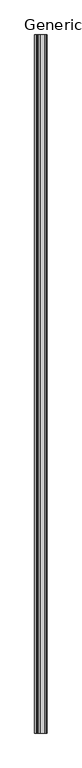
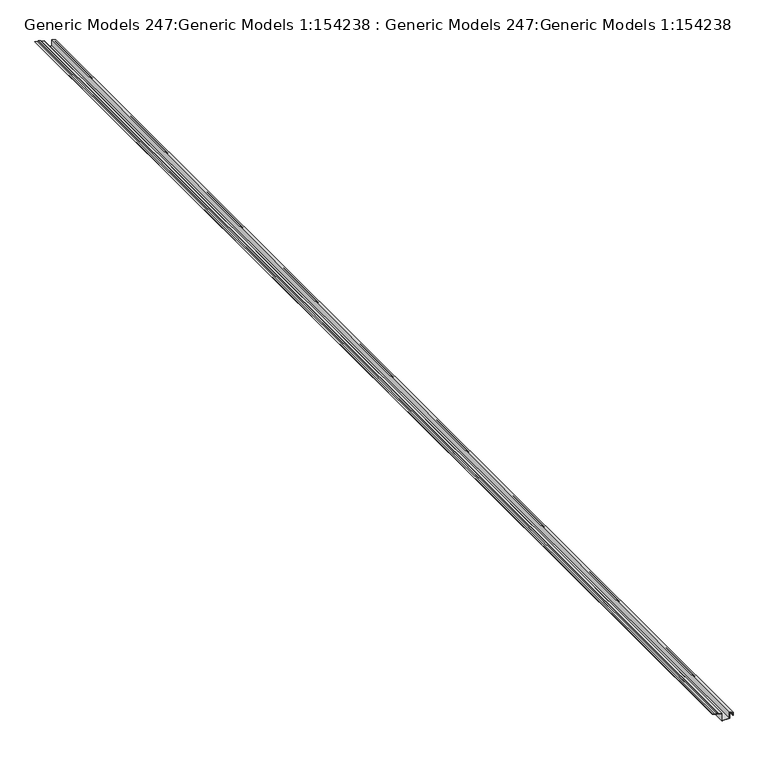
"""IFC4 building model written with IfcOpenShell, lengths in millimetres: proxy geometry, Generic Models 247:Generic Models 1:154238 : Generic Models 247:Generic Models 1:154238."""

from ifc_helpers import new_model, si_unit, point, frame, frame_2d, origin, place, context, project, spatial, polyline, circle_curve, trimmed, segment, composite_curve, outline, extrude, source, transform, mapped, element, save


def generic_models_247_generic_models_1_154238_generic_models_f81f4326(model_context):
    return source(origin(), model_context, "Body", "SweptSolid", [
        extrude(outline(polyline([(6352.8619087, 2093.6944594), (6358.1032399, 2089.5220922), (6375.8169733, 2089.5220922), (6375.8169733, 2087.9345922), (6357.5485246, 2087.9345922), (6352.3071934, 2092.1069594), (6332.0583841, 2092.1069594), (6332.0583841, 2093.6944594), (6352.8619087, 2093.6944594)])), frame((0.0, -1800.6402746, 0.0), z_axis=(0.0, 1.0, 0.0), x_axis=(0.0, 0.0, 1.0)), (0.0, 0.0, 1.0), 19050.0),
        extrude(outline(composite_curve([segment(polyline([(6442.7902622, 1834.0482885), (6438.1490188, 1852.6132622)]), True, "CONTINUOUS"), segment(trimmed(circle_curve(frame_2d((6442.2514638, 1853.6388734)), 4.2287035), [point((6438.1490188, 1852.6132622))], [point((6446.3539088, 1854.6644847))], False, "CARTESIAN"), True, "CONTINUOUS"), segment(polyline([(6446.3539088, 1854.6644847), (6455.0265499, 1819.9739201), (6448.9640649, 1798.1559096), (6457.809663, 1762.7735174), (6456.2695617, 1762.3884921), (6447.3223612, 1798.1772941), (6453.3848462, 1819.9953046), (6444.8138076, 1854.2794593)]), True, "CONTINUOUS"), segment(trimmed(circle_curve(frame_2d((6442.2064343, 1853.627616)), 2.6876188), [point((6444.8138076, 1854.2794593))], [point((6439.5990611, 1852.9757727))], True, "CARTESIAN"), True, "CONTINUOUS"), segment(polyline([(6439.5990611, 1852.9757727), (6444.2403045, 1834.4107991), (6442.7902622, 1834.0482885)]), True, "CONTINUOUS")], self_intersect=False)), frame((0.0, -1800.6402746, 0.0), z_axis=(0.0, 1.0, 0.0), x_axis=(0.0, 0.0, 1.0)), (0.0, 0.0, 1.0), 19050.0),
        extrude(outline(composite_curve([segment(polyline([(6393.669921, 2037.8396711), (6293.657421, 2037.8396711), (6293.657421, 1914.0146711), (6420.434256, 1914.0146711), (6441.5034772, 1829.7377864)]), True, "CONTINUOUS"), segment(trimmed(circle_curve(frame_2d((6444.4101981, 1830.4644666)), 2.9961793), [point((6441.5034772, 1829.7377864))], [point((6447.3169189, 1831.1911468))], True, "CARTESIAN"), True, "CONTINUOUS"), segment(polyline([(6447.3169189, 1831.1911468), (6441.9869213, 1852.5111372), (6443.5270226, 1852.8961625), (6448.8570202, 1831.5761721)]), True, "CONTINUOUS"), segment(trimmed(circle_curve(frame_2d((6444.4101981, 1830.4644666)), 4.5836793), [point((6448.8570202, 1831.5761721))], [point((6439.963376, 1829.3527611))], False, "CARTESIAN"), True, "CONTINUOUS"), segment(polyline([(6439.963376, 1829.3527611), (6419.1947735, 1912.4271711), (6292.069921, 1912.4271711), (6292.069921, 2039.4271711), (6391.6366884, 2039.4271711), (6377.6729546, 2095.2821066), (6332.6127313, 2095.2821066)]), True, "CONTINUOUS"), segment(trimmed(circle_curve(frame_2d((6332.6127313, 2093.1958494)), 2.0862572), [point((6332.6127313, 2095.2821066))], [point((6332.6127313, 2091.1095922))], True, "CARTESIAN"), True, "CONTINUOUS"), segment(polyline([(6332.6127313, 2091.1095922), (6347.8649537, 2091.1095922), (6347.8649537, 2089.5220922), (6332.6127313, 2089.5220922)]), True, "CONTINUOUS"), segment(trimmed(circle_curve(frame_2d((6332.6127313, 2093.1958494)), 3.6737572), [point((6332.6127313, 2089.5220922))], [point((6332.6127313, 2096.8696066))], False, "CARTESIAN"), True, "CONTINUOUS"), segment(polyline([(6332.6127313, 2096.8696066), (6378.9124371, 2096.8696066), (6393.669921, 2037.8396711)]), True, "CONTINUOUS")], self_intersect=False)), frame((0.0, -1800.6402746, 0.0), z_axis=(0.0, 1.0, 0.0), x_axis=(0.0, 0.0, 1.0)), (0.0, 0.0, 1.0), 19050.0),
    ])


if __name__ == "__main__":
    model = new_model("IFC4")
    model_context = context("Model", 3, world=origin())
    ifc_project = project(units=[si_unit("LENGTHUNIT", "METRE", prefix="MILLI")], contexts=[model_context])
    site = spatial("IfcSite", under=ifc_project)
    building = spatial("IfcBuilding", under=site)
    placement = place(None, origin())
    generic_models_247_generic_models_1_154238_generic_models_shape = generic_models_247_generic_models_1_154238_generic_models_f81f4326(model_context)
    element("IfcBuildingElementProxy", 1, Name="Generic Models 247:Generic Models 1:154238 : Generic Models 247:Generic Models 1:154238", ObjectType="Generic Models 247:Generic Models 1:154238 : Generic Models 247:Generic Models 1:154238", at=placement, inside=building, context=model_context, shape_type="MappedRepresentation", body=[
        mapped(generic_models_247_generic_models_1_154238_generic_models_shape, transform((0.0, 0.0, 0.0), x_axis=(1.0, 0.0, 0.0), y_axis=(0.0, 1.0, 0.0), z_axis=(0.0, 0.0, 1.0))),
    ])
    save(model, "model.ifc")

# Revit data of these elements
# Type "Generic Models 247:Generic Models 1:154238 : Generic Models 247:Generic Models 1:154238"
#   NameOverride = "Generic Models 247:Generic Models 1:154238"
#   ObjectTypeOverride = "Generic Models 247:Generic Models 1"
#   Reference = "Generic Models 1"
#   Category = "Generic Models"
#   Tag = "154238"
# Element 1 (IfcBuildingElementProxy, "Generic Models 247:Generic Models 1:154238 : Generic Models 247:Generic Models 1:154238")
#   Materials on its faces: "_CONT. SEAMLESS BRAKE METAL GUTTER 21235"
# Materials
#   "_CONT. SEAMLESS BRAKE METAL GUTTER 21235": class "Unassigned", colour RGB 175 175 175, transparency 0
